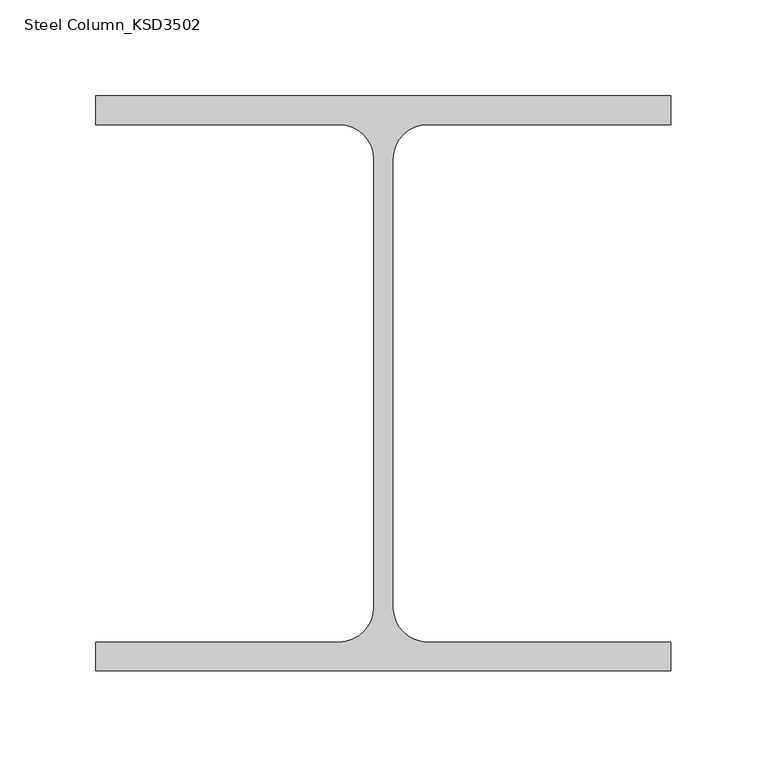
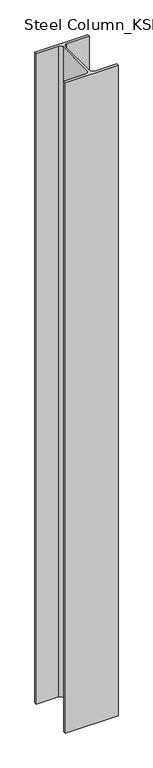
"""IFC4 building model written with IfcOpenShell, lengths in millimetres: column geometry, Steel Column_KSD3502 : H_SC_ASC_H-300×300x10x15."""

from ifc_helpers import new_model, si_unit, point, frame, frame_2d, origin, place, context, project, spatial, polyline, circle_curve, trimmed, segment, composite_curve, outline, extrude, source, transform, mapped, element, save


def steel_column_ksd3502_599e6a97(model_context):
    return source(origin(), model_context, "Body", "SweptSolid", [
        extrude(outline(composite_curve([segment(polyline([(150.0, 150.0), (150.0, 135.0), (23.0, 135.0)]), True, "CONTINUOUS"), segment(trimmed(circle_curve(frame_2d((23.0, 117.0)), 18.0), [point((23.0, 135.0))], [point((5.0, 117.0))], True, "CARTESIAN"), True, "CONTINUOUS"), segment(polyline([(5.0, 117.0), (5.0, -117.0)]), True, "CONTINUOUS"), segment(trimmed(circle_curve(frame_2d((23.0, -117.0)), 18.0), [point((5.0, -117.0))], [point((23.0, -135.0))], True, "CARTESIAN"), True, "CONTINUOUS"), segment(polyline([(23.0, -135.0), (150.0, -135.0), (150.0, -150.0), (-150.0, -150.0), (-150.0, -135.0), (-23.0, -135.0)]), True, "CONTINUOUS"), segment(trimmed(circle_curve(frame_2d((-23.0, -117.0)), 18.0), [point((-23.0, -135.0))], [point((-5.0, -117.0))], True, "CARTESIAN"), True, "CONTINUOUS"), segment(polyline([(-5.0, -117.0), (-5.0, 117.0)]), True, "CONTINUOUS"), segment(trimmed(circle_curve(frame_2d((-23.0, 117.0)), 18.0), [point((-5.0, 117.0))], [point((-23.0, 135.0))], True, "CARTESIAN"), True, "CONTINUOUS"), segment(polyline([(-23.0, 135.0), (-150.0, 135.0), (-150.0, 150.0), (150.0, 150.0)]), True, "CONTINUOUS")], self_intersect=False)), frame((0.0, 0.0, 685.9720055), z_axis=(0.0, 0.0, 1.0), x_axis=(1.0, 0.0, 0.0)), (0.0, 0.0, 1.0), 3914.0),
    ])


if __name__ == "__main__":
    model = new_model("IFC4")
    model_context = context("Model", 3, world=origin())
    ifc_project = project(units=[si_unit("LENGTHUNIT", "METRE", prefix="MILLI")], contexts=[model_context])
    site = spatial("IfcSite", under=ifc_project)
    building = spatial("IfcBuilding", under=site)
    placement = place(None, origin())
    steel_column_ksd3502_shape = steel_column_ksd3502_599e6a97(model_context)
    element("IfcColumn", 1, ObjectType="Steel Column_KSD3502 : H_SC_ASC_H-300×300x10x15", at=placement, inside=building, context=model_context, shape_type="MappedRepresentation", body=[
        mapped(steel_column_ksd3502_shape, transform((0.0, 0.0, 0.0), x_axis=(1.0, 0.0, 0.0), y_axis=(0.0, 1.0, 0.0), z_axis=(0.0, 0.0, 1.0))),
    ])
    save(model, "model.ifc")

# Revit data of these elements
# Type "Steel Column_KSD3502 : H_SC_ASC_H-300×300x10x15"
#   Width = 30.0 cm
#   Web Thickness = 1.0 cm
#   Web Fillet = 1.8 cm
#   Warping Constant = 1370670.0 cm⁶
#   Torsional Moment of Inertia = 77.00 cm⁴
#   Section Area = 119.8 cm²
#   Plastic Modulus weak axis = 684.0 cm³
#   Plastic Modulus strong axis = 1500.0 cm³
#   Perimeter = 1.27 m²/m
#   Nominal Weight = 94.00 kgf/m
#   Moment of Inertia weak axis = 6750.00 cm⁴
#   Moment of Inertia strong axis = 20400.00 cm⁴
#   Height = 30.0 cm
#   Flange Thickness = 1.5 cm
#   Elastic Modulus weak axis = 450.0 cm³
#   Elastic Modulus strong axis = 1360.0 cm³
#   Centroid Vertical = 15.0 cm
#   Centroid Horizontal = 15.0 cm
#   Bolt Spacing = 13.97 cm
#   Structural Material [instance default] = Steel, 45-345
#   Section Name Key = ""
#   Assembly Code = ""
# Element 1 (IfcColumn, "Steel Column_KSD3502 : H_SC_ASC_H-300×300x10x15")
#   Structural Material = none
# Materials
#   "Steel, 45-345": class "Metal", colour RGB 189 187 185, transparency 0, Description = "Steel 345 MPa", Cost = 0
